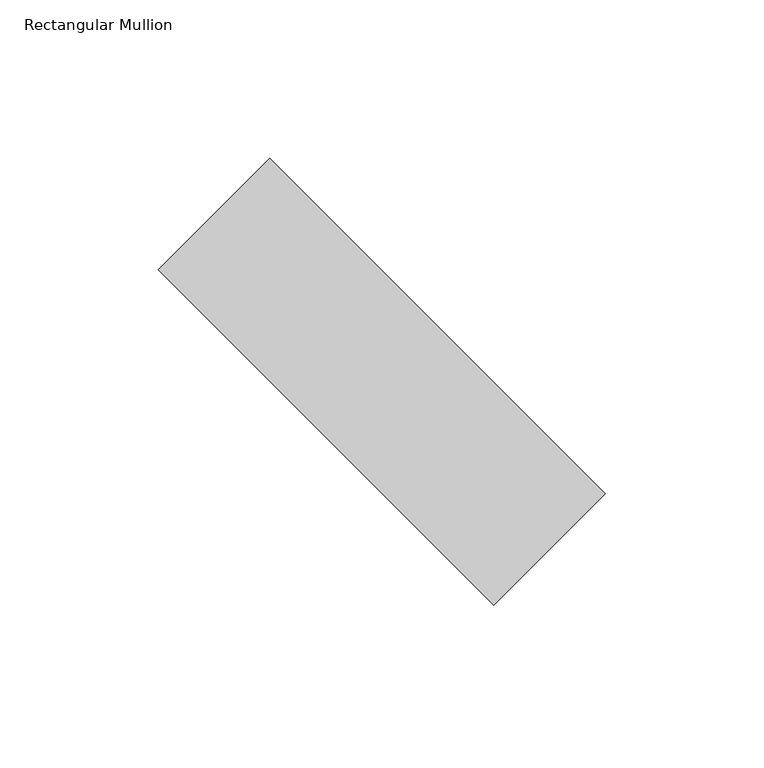
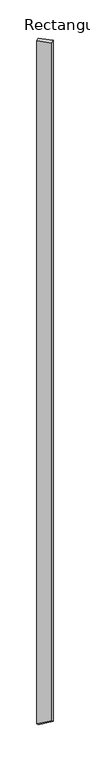
"""IFC4 building model written with IfcOpenShell, lengths in millimetres: member geometry, Rectangular Mullion : tilted mullions."""

from ifc_helpers import new_model, si_unit, origin, place, context, project, spatial, faceted_brep, source, transform, mapped, element, save


def rectangular_mullion_2c8bbd53(model_context):
    return source(origin(), model_context, "Body", "Brep", [
        faceted_brep([(-35.3553391, 70.7106781, 0.0), (-70.7106781, 35.3553391, 0.0), (35.3553391, -70.7106781, 0.0), (70.7106781, -35.3553391, 0.0), (-35.3553391, 70.7106781, -8054.3689422), (-70.7106781, 35.3553391, -8009.3419618), (35.3553391, -70.7106781, -7944.1258646), (70.7106781, -35.3553391, -7989.152845)], [[[0, 1, 2, 3]], [[1, 0, 4, 5]], [[2, 1, 5, 6]], [[3, 2, 6, 7]], [[0, 3, 7, 4]], [[4, 7, 6, 5]]]),
    ])


if __name__ == "__main__":
    model = new_model("IFC4")
    model_context = context("Model", 3, world=origin())
    ifc_project = project(units=[si_unit("LENGTHUNIT", "METRE", prefix="MILLI")], contexts=[model_context])
    site = spatial("IfcSite", under=ifc_project)
    building = spatial("IfcBuilding", under=site)
    placement = place(None, origin())
    rectangular_mullion_shape = rectangular_mullion_2c8bbd53(model_context)
    element("IfcMember", 1, ObjectType="Rectangular Mullion : tilted mullions", at=placement, inside=building, context=model_context, shape_type="MappedRepresentation", body=[
        mapped(rectangular_mullion_shape, transform((0.0, 0.0, 0.0), x_axis=(1.0, 0.0, 0.0), y_axis=(0.0, 1.0, 0.0), z_axis=(0.0, 0.0, 1.0))),
    ])
    save(model, "model.ifc")

# Revit data of these elements
# Type "Rectangular Mullion : tilted mullions"
#   built-in parameter 1007304 = 0.492126 (stored number, unit not read)
#   built-in parameter 1007301 = 0.082021 (stored number, unit not read)
#   built-in parameter 1007300 = 0.082021 (stored number, unit not read)
# Element 1 (IfcMember, "Rectangular Mullion : tilted mullions")
#   Materials on its faces: "Aluminum"
# Materials
#   "Aluminum": class "Metal", colour RGB 244 244 244, transparency 0, Description = "Aluminum 6061", Cost = 0
